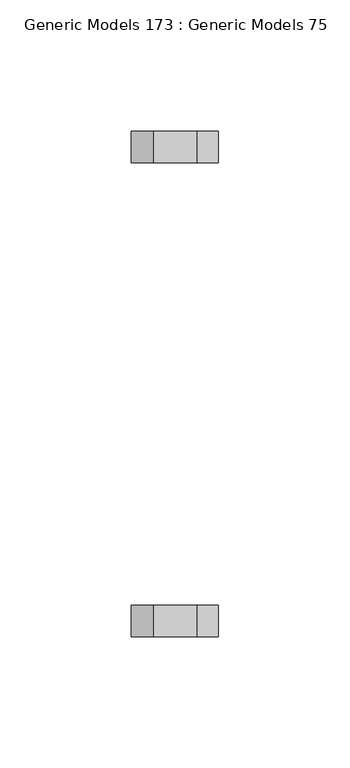
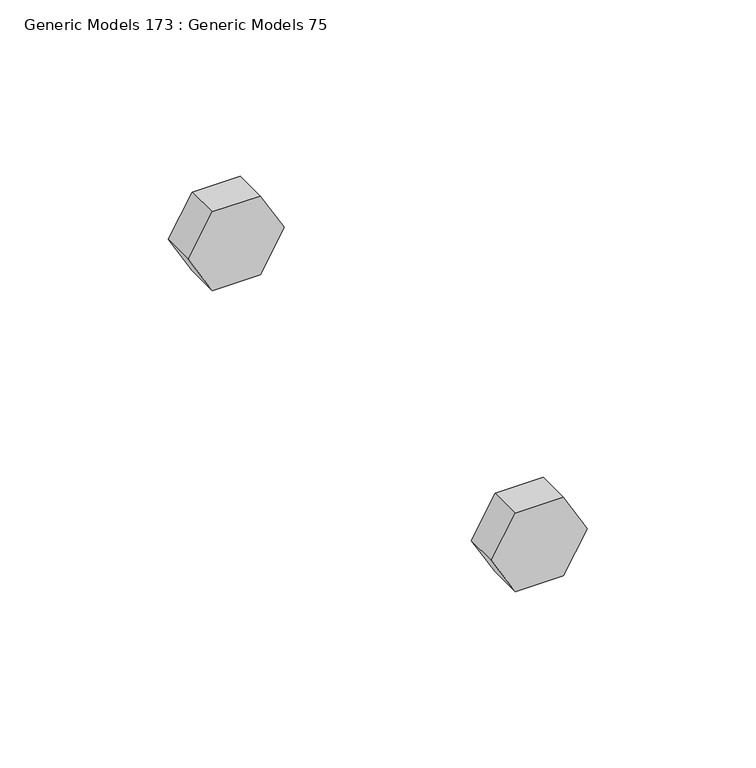
"""IFC4 building model written with IfcOpenShell, lengths in millimetres: proxy geometry, Generic Models 173 : Generic Models 75."""

from ifc_helpers import new_model, si_unit, frame, origin, place, context, project, spatial, polyline, outline, extrude, source, transform, mapped, element, save


def generic_models_173_generic_models_75_790f61a9(model_context):
    return source(origin(), model_context, "Body", "SweptSolid", [
        extrude(outline(polyline([(271581.5625, 31978.2851858), (271581.5625, 31994.7829698), (271595.85, 32003.0318618), (271610.1375, 31994.7829698), (271610.1375, 31978.2851858), (271595.85, 31970.0362939), (271581.5625, 31978.2851858)])), frame((0.0, 35193.7770442, 0.0), z_axis=(0.0, 1.0, 0.0), x_axis=(0.0, 0.0, 1.0)), (0.0, 0.0, 1.0), 11.90625),
        extrude(outline(polyline([(271581.5625, 31978.2851858), (271581.5625, 31994.7829698), (271595.85, 32003.0318618), (271610.1375, 31994.7829698), (271610.1375, 31978.2851858), (271595.85, 31970.0362939), (271581.5625, 31978.2851858)])), frame((0.0, 35373.9582942, 0.0), z_axis=(0.0, 1.0, 0.0), x_axis=(0.0, 0.0, 1.0)), (0.0, 0.0, 1.0), 11.90625),
    ])


if __name__ == "__main__":
    model = new_model("IFC4")
    model_context = context("Model", 3, world=origin())
    ifc_project = project(units=[si_unit("LENGTHUNIT", "METRE", prefix="MILLI")], contexts=[model_context])
    site = spatial("IfcSite", under=ifc_project)
    building = spatial("IfcBuilding", under=site)
    placement = place(None, origin())
    generic_models_173_generic_models_75_shape = generic_models_173_generic_models_75_790f61a9(model_context)
    element("IfcBuildingElementProxy", 1, Name="Generic Models 173 : Generic Models 75", ObjectType="Generic Models 173 : Generic Models 75", at=placement, inside=building, context=model_context, shape_type="MappedRepresentation", body=[
        mapped(generic_models_173_generic_models_75_shape, transform((0.0, 0.0, 0.0), x_axis=(1.0, 0.0, 0.0), y_axis=(0.0, 1.0, 0.0), z_axis=(0.0, 0.0, 1.0))),
    ])
    save(model, "model.ifc")

# Revit data of these elements
# Element 1 (IfcBuildingElementProxy, "Generic Models 173 : Generic Models 75")
#   Materials on its faces: "3/4\" GALV. THRU BOLTS"
# Materials
#   "3/4\" GALV. THRU BOLTS": class "Generic", colour RGB 105 69 171, transparency 0, Cost = 0
